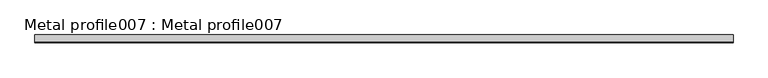
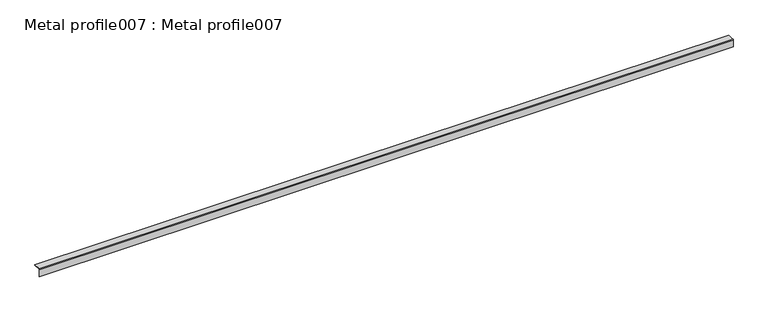
"""IFC4 building model written with IfcOpenShell, lengths in millimetres: proxy geometry, Metal profile007 : Metal profile007."""

from ifc_helpers import new_model, si_unit, point, frame, frame_2d, origin, place, context, project, spatial, polyline, circle_curve, trimmed, segment, composite_curve, outline, extrude, source, transform, mapped, element, save


def metal_profile007_metal_profile007_183138f6(model_context):
    return source(origin(), model_context, "Body", "SweptSolid", [
        extrude(outline(composite_curve([segment(polyline([(9598.7832673, 37512.0598437), (9577.6300834, 37512.0598437), (9577.6300834, 37490.9066598), (9576.3500834, 37490.9066598), (9576.3500834, 37511.8095695)]), True, "CONTINUOUS"), segment(trimmed(circle_curve(frame_2d((9576.9900834, 37512.6998437)), 1.0964434), [point((9576.3500834, 37511.8095695))], [point((9577.8803576, 37513.3398437))], False, "CARTESIAN"), True, "CONTINUOUS"), segment(polyline([(9577.8803576, 37513.3398437), (9598.7832673, 37513.3398437), (9598.7832673, 37512.0598437)]), True, "CONTINUOUS")], self_intersect=False)), frame((3694.2883192, 0.0, 0.0), z_axis=(1.0, 0.0, 0.0), x_axis=(0.0, 1.0, 0.0)), (0.0, 0.0, 1.0), 2000.0),
    ])


if __name__ == "__main__":
    model = new_model("IFC4")
    model_context = context("Model", 3, world=origin())
    ifc_project = project(units=[si_unit("LENGTHUNIT", "METRE", prefix="MILLI")], contexts=[model_context])
    site = spatial("IfcSite", under=ifc_project)
    building = spatial("IfcBuilding", under=site)
    placement = place(None, origin())
    metal_profile007_metal_profile007_shape = metal_profile007_metal_profile007_183138f6(model_context)
    element("IfcBuildingElementProxy", 1, Name="Metal profile007 : Metal profile007", ObjectType="Metal profile007 : Metal profile007", at=placement, inside=building, context=model_context, shape_type="MappedRepresentation", body=[
        mapped(metal_profile007_metal_profile007_shape, transform((0.0, 0.0, 0.0), x_axis=(1.0, 0.0, 0.0), y_axis=(0.0, 1.0, 0.0), z_axis=(0.0, 0.0, 1.0))),
    ])
    save(model, "model.ifc")

# Revit data of these elements
# Type "Metal profile007 : Metal profile007"
#   NameOverride = "Metal profile007"
# Element 1 (IfcBuildingElementProxy, "Metal profile007 : Metal profile007")
#   Materials on its faces: "CORNER BEAD"
# Materials
#   "CORNER BEAD": class "Unassigned", colour RGB 253 236 176, transparency 0, Cost = 0
